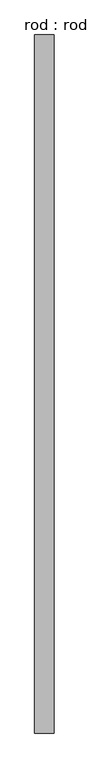
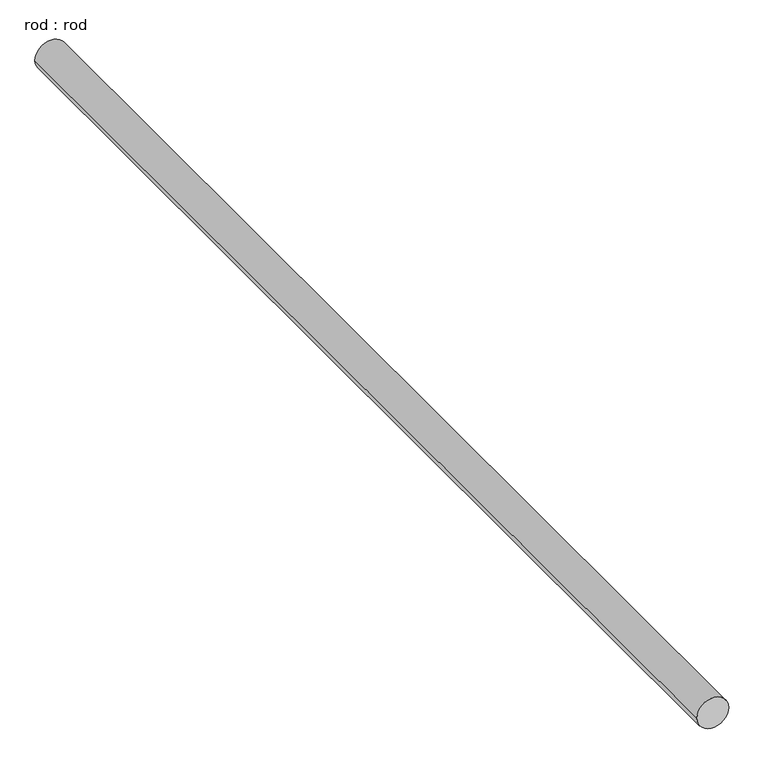
"""IFC4 building model written with IfcOpenShell, lengths in millimetres: proxy geometry, rod : rod."""

from ifc_helpers import new_model, si_unit, point, frame, frame_2d, origin, place, context, project, spatial, circle_curve, trimmed, segment, composite_curve, outline, extrude, source, transform, mapped, element, save


def rod_rod_9c033583(model_context):
    return source(origin(), model_context, "Body", "SweptSolid", [
        extrude(outline(composite_curve([segment(trimmed(circle_curve(frame_2d((0.0108462, 0.0)), 200.0), [point((0.0108462, 200.0))], [point((0.0108462, -200.0))], False, "CARTESIAN"), True, "CONTINUOUS"), segment(trimmed(circle_curve(frame_2d((0.0108462, 0.0)), 200.0), [point((0.0108462, -200.0))], [point((0.0108462, 200.0))], False, "CARTESIAN"), True, "CONTINUOUS")], self_intersect=False)), frame((0.0, -3107.2713847, 0.0), z_axis=(0.0, 1.0, 0.0), x_axis=(0.0, 0.0, 1.0)), (0.0, 0.0, 1.0), 14400.0),
    ])


if __name__ == "__main__":
    model = new_model("IFC4")
    model_context = context("Model", 3, world=origin())
    ifc_project = project(units=[si_unit("LENGTHUNIT", "METRE", prefix="MILLI")], contexts=[model_context])
    site = spatial("IfcSite", under=ifc_project)
    building = spatial("IfcBuilding", under=site)
    placement = place(None, origin())
    rod_rod_shape = rod_rod_9c033583(model_context)
    element("IfcBuildingElementProxy", 1, Name="rod : rod", ObjectType="rod : rod", at=placement, inside=building, context=model_context, shape_type="MappedRepresentation", body=[
        mapped(rod_rod_shape, transform((0.0, 0.0, 0.0), x_axis=(1.0, 0.0, 0.0), y_axis=(0.0, 1.0, 0.0), z_axis=(0.0, 0.0, 1.0))),
    ])
    save(model, "model.ifc")

# Revit data of these elements
# Type "rod : rod"
#   Default Elevation = 0
